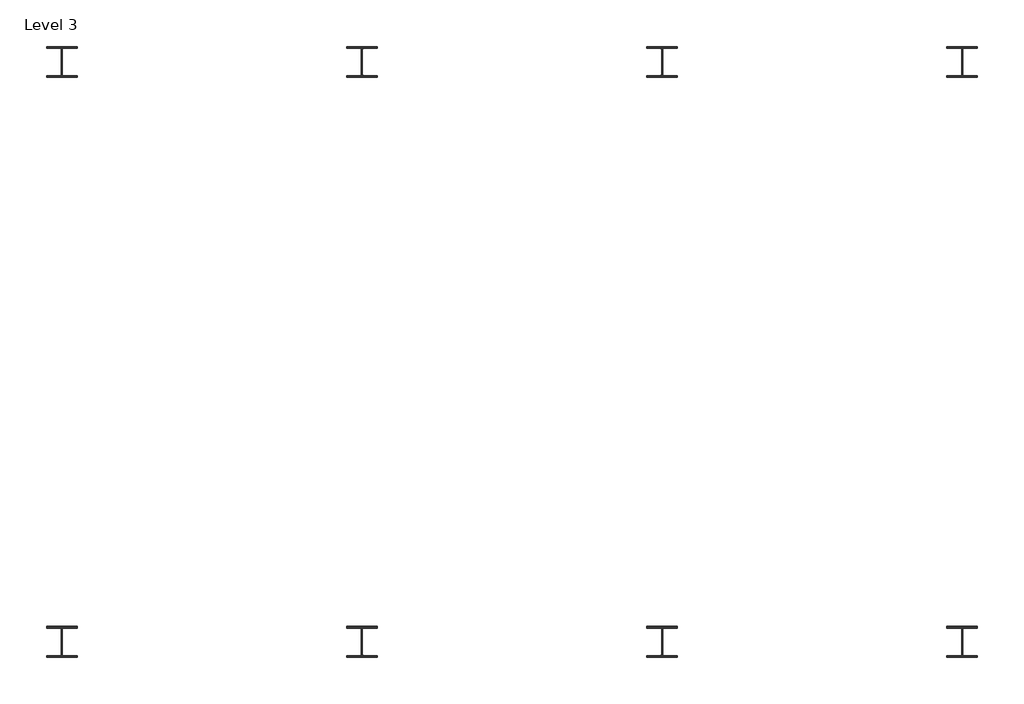
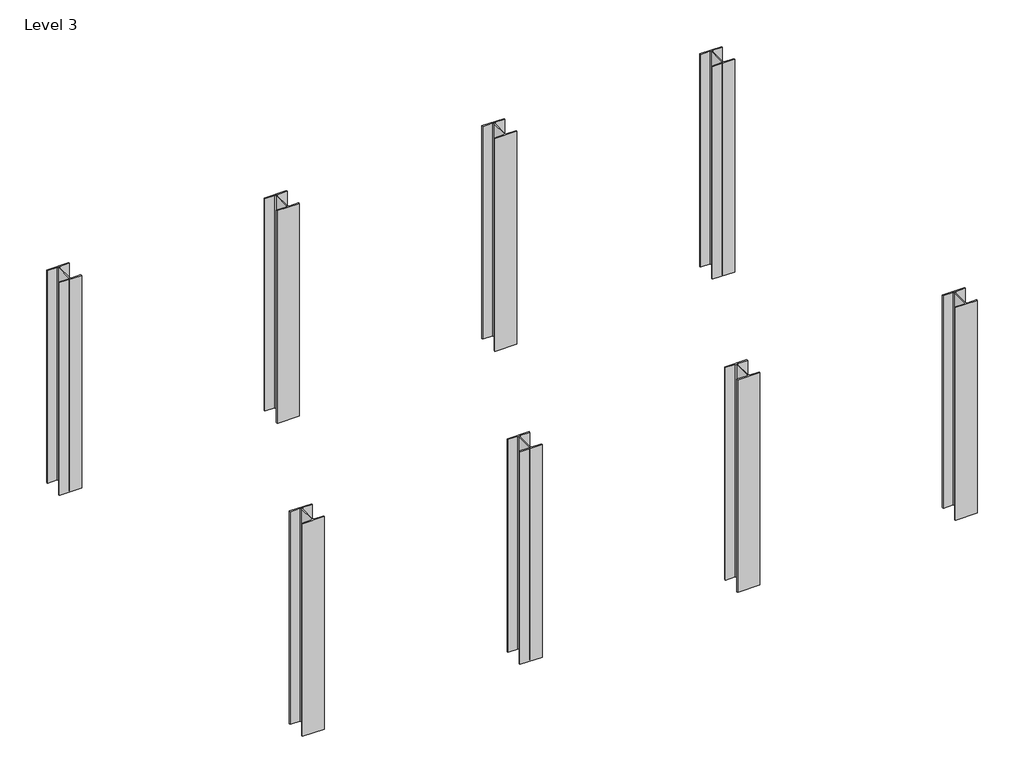
# One storey: 8 columns.
"""IFC4 building model written with IfcOpenShell, lengths in millimetres."""

import ifcopenshell
import ifcopenshell.guid

model = None  # the IFC model being written
_history = None  # IfcOwnerHistory: only IFC2X3 demands one
_inside = {}  # id of a spatial element -> (the spatial element, [elements in it])
_under = {}  # id of a project, library or spatial element -> (it, [spatial elements below it])
_declared = {}  # id of a project -> (the project, [libraries it declares])
_typed = {}  # id of a type object -> (the type object, [elements of that type])
_made_of = {}  # id of a material, layer set ... -> (it, [elements and type objects made of it])


def new_model(schema):
    """Start an empty IFC model of exactly this schema.

    Asked for "IFC4X3", IfcOpenShell would pick the latest addendum, in which some entities
    have other attributes; the version numbers below select the first issue.
    IFC2X3 requires an IfcOwnerHistory on every rooted entity: one is made here for all.
    """
    global model, _history
    if schema == "IFC4X3":
        model = ifcopenshell.file(schema_version=(4, 3, 0, 0))
    else:
        model = ifcopenshell.file(schema=schema)
    _inside.clear()
    _under.clear()
    _declared.clear()
    _typed.clear()
    _made_of.clear()
    _history = None
    if model.schema == "IFC2X3":
        org = make("IfcOrganization", Name="unknown")
        user = make(
            "IfcPersonAndOrganization",
            ThePerson=make("IfcPerson", FamilyName="unknown"),
            TheOrganization=org,
        )
        app = make(
            "IfcApplication",
            ApplicationDeveloper=org,
            Version="unknown",
            ApplicationFullName="unknown",
            ApplicationIdentifier="unknown",
        )
        _history = make(
            "IfcOwnerHistory",
            OwningUser=user,
            OwningApplication=app,
            ChangeAction="ADDED",
            CreationDate=0,
        )
    return model


def make(cls, **values):
    """One entity of the class cls with the attributes given. An attribute that is None is left unset."""
    return model.create_entity(
        cls, **{name: value for name, value in values.items() if value is not None}
    )


def rooted(cls, **values):
    """An entity with a GlobalId (a new one), such as an element, a storey or a relation."""
    return make(cls, GlobalId=ifcopenshell.guid.new(), OwnerHistory=_history, **values)


def si_unit(unit_type, name, prefix=None):
    """IfcSIUnit, for example si_unit("LENGTHUNIT", "METRE", prefix="MILLI")."""
    return make("IfcSIUnit", UnitType=unit_type, Prefix=prefix, Name=name)


def assignment(units):
    """IfcUnitAssignment: the units of a project."""
    return None if units is None else make("IfcUnitAssignment", Units=units)


def point(xyz):
    """IfcCartesianPoint."""
    return None if xyz is None else make("IfcCartesianPoint", Coordinates=xyz)


def direction(xyz):
    """IfcDirection."""
    return None if xyz is None else make("IfcDirection", DirectionRatios=xyz)


def frame(location, z_axis=None, x_axis=None):
    """IfcAxis2Placement3D, a coordinate frame: its origin and axes. An axis left out is left unset."""
    return make(
        "IfcAxis2Placement3D",
        Location=point(location),
        Axis=direction(z_axis),
        RefDirection=direction(x_axis),
    )


def frame_2d(location, x_axis=None):
    """IfcAxis2Placement2D, a coordinate frame in the plane: its origin and x axis."""
    return make(
        "IfcAxis2Placement2D", Location=point(location), RefDirection=direction(x_axis)
    )


def origin():
    """The frame at (0, 0, 0) with its axes left unset."""
    return frame((0.0, 0.0, 0.0))


def place(relative_to, where):
    """IfcLocalPlacement: puts the frame where relative to a parent placement (None: the world)."""
    return make(
        "IfcLocalPlacement", PlacementRelTo=relative_to, RelativePlacement=where
    )


def context(
    kind, dimensions, precision=None, world=None, true_north=None, identifier=None
):
    """IfcGeometricRepresentationContext, for example the 3D "Model" context."""
    return make(
        "IfcGeometricRepresentationContext",
        ContextIdentifier=identifier,
        ContextType=kind,
        CoordinateSpaceDimension=dimensions,
        Precision=precision,
        WorldCoordinateSystem=world,
        TrueNorth=true_north,
    )


def project(units=None, contexts=None):
    """IfcProject with its units and contexts."""
    return rooted(
        "IfcProject",
        Name="project",
        RepresentationContexts=contexts,
        UnitsInContext=assignment(units),
    )


def spatial(cls, under=None, at=None, **own):
    """A site, building, storey or space (cls), placed at a placement, below another one or the project."""
    s = rooted(cls, ObjectPlacement=at, **own)
    if under is not None:
        _under.setdefault(under.id(), (under, []))[1].append(s)
    return s


def polyline(points):
    """IfcPolyline through the points."""
    return make("IfcPolyline", Points=[point(p) for p in points])


def circle_curve(where, radius):
    """IfcCircle in the frame where."""
    return make("IfcCircle", Position=where, Radius=radius)


def trimmed(basis, trim1, trim2, sense, master):
    """IfcTrimmedCurve: the piece of a basis curve between two trims."""
    return make(
        "IfcTrimmedCurve",
        BasisCurve=basis,
        Trim1=trim1,
        Trim2=trim2,
        SenseAgreement=sense,
        MasterRepresentation=master,
    )


def segment(curve, same_sense, transition):
    """IfcCompositeCurveSegment."""
    return make(
        "IfcCompositeCurveSegment",
        Transition=transition,
        SameSense=same_sense,
        ParentCurve=curve,
    )


def composite_curve(segments, self_intersect=None):
    """IfcCompositeCurve: segments joined end to end."""
    return make("IfcCompositeCurve", Segments=segments, SelfIntersect=self_intersect)


def outline(outer, holes=None, kind="AREA"):
    """IfcArbitraryClosedProfileDef: a profile drawn as a closed curve; with holes, ...WithVoids."""
    if holes is None:
        return make("IfcArbitraryClosedProfileDef", ProfileType=kind, OuterCurve=outer)
    return make(
        "IfcArbitraryProfileDefWithVoids",
        ProfileType=kind,
        OuterCurve=outer,
        InnerCurves=holes,
    )


def extrude(swept, where, along, depth):
    """IfcExtrudedAreaSolid: the profile swept, set in the frame where, extruded along a direction by depth."""
    return make(
        "IfcExtrudedAreaSolid",
        SweptArea=swept,
        Position=where,
        ExtrudedDirection=direction(along),
        Depth=depth,
    )


def shape(context_of_items, identifier, shape_type, items):
    """IfcShapeRepresentation: the items that make up one representation, for example the "Body"."""
    return make(
        "IfcShapeRepresentation",
        ContextOfItems=context_of_items,
        RepresentationIdentifier=identifier,
        RepresentationType=shape_type,
        Items=items,
    )


def source(mapping_origin, context_of_items, identifier, shape_type, items):
    """IfcRepresentationMap: a shape defined once, which mapped items show again and again."""
    return make(
        "IfcRepresentationMap",
        MappingOrigin=mapping_origin,
        MappedRepresentation=shape(context_of_items, identifier, shape_type, items),
    )


def transform(
    local_origin,
    x_axis=None,
    y_axis=None,
    z_axis=None,
    scale=None,
    scale2=None,
    scale3=None,
    uniform=True,
):
    """IfcCartesianTransformationOperator3D, or its non-uniform kind. x_axis, y_axis, z_axis: its Axis1, 2, 3."""
    if uniform:
        return make(
            "IfcCartesianTransformationOperator3D",
            Axis1=direction(x_axis),
            Axis2=direction(y_axis),
            LocalOrigin=point(local_origin),
            Scale=scale,
            Axis3=direction(z_axis),
        )
    return make(
        "IfcCartesianTransformationOperator3DnonUniform",
        Axis1=direction(x_axis),
        Axis2=direction(y_axis),
        LocalOrigin=point(local_origin),
        Scale=scale,
        Axis3=direction(z_axis),
        Scale2=scale2,
        Scale3=scale3,
    )


def mapped(mapping_source, mapping_target):
    """IfcMappedItem: shows the shape of a source again, moved by a transform."""
    return make(
        "IfcMappedItem", MappingSource=mapping_source, MappingTarget=mapping_target
    )


def made_of(thing, what):
    """Note that an element or type object is made of a material, layer set ...; save() writes the relation."""
    if what is not None:
        _made_of.setdefault(what.id(), (what, []))[1].append(thing)
    return thing


def element(
    cls,
    number,
    at=None,
    inside=None,
    cuts=None,
    type_object=None,
    material=None,
    context=None,
    identifier="Body",
    shape_type=None,
    held_by="IfcProductDefinitionShape",
    body=None,
    shapes=None,
    **own,
):
    """One element of the class cls, such as IfcWall. Its Tag is "e" and its number.

    at: its placement. inside: the storey or other place that contains it. cuts: it is an
    opening in that element (IfcRelVoidsElement). A single representation is given by context,
    identifier, shape_type and body (its items); several are given by shapes. held_by: the class
    of the entity that holds the representations. save() writes the other relations.
    """
    e = rooted(cls, Tag="e%d" % number, ObjectPlacement=at, **own)
    if body is not None:
        shapes = [shape(context, identifier, shape_type, body)]
    if shapes is not None:
        e.Representation = make(held_by, Representations=shapes)
    if inside is not None:
        _inside.setdefault(inside.id(), (inside, []))[1].append(e)
    if cuts is not None:
        rooted(
            "IfcRelVoidsElement", RelatingBuildingElement=cuts, RelatedOpeningElement=e
        )
    if type_object is not None:
        _typed.setdefault(type_object.id(), (type_object, []))[1].append(e)
    return made_of(e, material)


def aggregate(whole, parts):
    """IfcRelAggregates: a whole, such as a stair, and the parts it consists of."""
    return rooted("IfcRelAggregates", RelatingObject=whole, RelatedObjects=parts)


def save(model, path):
    """Write the relations noted so far, then the file.

    IfcRelAggregates (storeys below a building ...), IfcRelContainedInSpatialStructure (elements
    in a storey), IfcRelDefinesByType, IfcRelAssociatesMaterial and IfcRelDeclares: one each for
    every whole, place, type object, material and project.
    """
    for whole, parts in _under.values():
        aggregate(whole, parts)
    for where, things in _inside.values():
        rooted(
            "IfcRelContainedInSpatialStructure",
            RelatedElements=things,
            RelatingStructure=where,
        )
    for kind, things in _typed.values():
        rooted("IfcRelDefinesByType", RelatedObjects=things, RelatingType=kind)
    for what, things in _made_of.values():
        rooted("IfcRelAssociatesMaterial", RelatedObjects=things, RelatingMaterial=what)
    for by, libraries in _declared.values():
        rooted("IfcRelDeclares", RelatingContext=by, RelatedDefinitions=libraries)
    model.write(path)


def uc_universal_columns_column_uc305x305x97_b067ee91(model_context):
    return source(origin(), model_context, "Body", "SweptSolid", [
        extrude(outline(composite_curve([segment(polyline([(152.65, 153.95), (152.65, 138.55), (20.15, 138.55)]), True, "CONTINUOUS"), segment(trimmed(circle_curve(frame_2d((20.15, 123.35)), 15.2), [point((20.15, 138.55))], [point((4.95, 123.35))], True, "CARTESIAN"), True, "CONTINUOUS"), segment(polyline([(4.95, 123.35), (4.95, -123.35)]), True, "CONTINUOUS"), segment(trimmed(circle_curve(frame_2d((20.15, -123.35)), 15.2), [point((4.95, -123.35))], [point((20.15, -138.55))], True, "CARTESIAN"), True, "CONTINUOUS"), segment(polyline([(20.15, -138.55), (152.65, -138.55), (152.65, -153.95), (-152.65, -153.95), (-152.65, -138.55), (-20.15, -138.55)]), True, "CONTINUOUS"), segment(trimmed(circle_curve(frame_2d((-20.15, -123.35)), 15.2), [point((-20.15, -138.55))], [point((-4.95, -123.35))], True, "CARTESIAN"), True, "CONTINUOUS"), segment(polyline([(-4.95, -123.35), (-4.95, 123.35)]), True, "CONTINUOUS"), segment(trimmed(circle_curve(frame_2d((-20.15, 123.35)), 15.2), [point((-4.95, 123.35))], [point((-20.15, 138.55))], True, "CARTESIAN"), True, "CONTINUOUS"), segment(polyline([(-20.15, 138.55), (-152.65, 138.55), (-152.65, 153.95), (152.65, 153.95)]), True, "CONTINUOUS")], self_intersect=False)), frame((0.0, 0.0, 2900.0), z_axis=(0.0, 0.0, 1.0), x_axis=(1.0, 0.0, 0.0)), (0.0, 0.0, 1.0), 3100.0),
    ])


model = new_model("IFC4")

# Units and contexts
model_context = context("Model", 3, world=origin())
ifc_project = project(units=[si_unit("LENGTHUNIT", "METRE", prefix="MILLI")], contexts=[model_context])

# Site, building, storey
site = spatial("IfcSite", under=ifc_project)
building = spatial("IfcBuilding", under=site)
storey = spatial("IfcBuildingStorey", under=building, Name="Level 3", Elevation=3000.0)

# Columns
placement = place(None, origin())
uc_universal_columns_column_uc305x305x97_shape = uc_universal_columns_column_uc305x305x97_b067ee91(model_context)
element("IfcColumn", 1, ObjectType="UC-Universal Columns-Column : UC305x305x97", at=placement, inside=storey, context=model_context, shape_type="MappedRepresentation", body=[
    mapped(uc_universal_columns_column_uc305x305x97_shape, transform((-1938.0684826, 2696.9060214, 0.0), x_axis=(-1.0, 0.0, 0.0), y_axis=(0.0, -1.0, 0.0), z_axis=(0.0, 0.0, 1.0))),
])
element("IfcColumn", 2, ObjectType="UC-Universal Columns-Column : UC305x305x97", at=placement, inside=storey, context=model_context, shape_type="MappedRepresentation", body=[
    mapped(uc_universal_columns_column_uc305x305x97_shape, transform((-1938.0684826, -3100.0939786, 0.0), x_axis=(-1.0, 0.0, 0.0), y_axis=(0.0, -1.0, 0.0), z_axis=(0.0, 0.0, 1.0))),
])
element("IfcColumn", 3, ObjectType="UC-Universal Columns-Column : UC305x305x97", at=placement, inside=storey, context=model_context, shape_type="MappedRepresentation", body=[
    mapped(uc_universal_columns_column_uc305x305x97_shape, transform((1061.9315174, 2696.9060214, 0.0), x_axis=(-1.0, 0.0, 0.0), y_axis=(0.0, -1.0, 0.0), z_axis=(0.0, 0.0, 1.0))),
])
element("IfcColumn", 4, ObjectType="UC-Universal Columns-Column : UC305x305x97", at=placement, inside=storey, context=model_context, shape_type="MappedRepresentation", body=[
    mapped(uc_universal_columns_column_uc305x305x97_shape, transform((1061.9315174, -3100.0939786, 0.0), x_axis=(-1.0, 0.0, 0.0), y_axis=(0.0, -1.0, 0.0), z_axis=(0.0, 0.0, 1.0))),
])
element("IfcColumn", 5, ObjectType="UC-Universal Columns-Column : UC305x305x97", at=placement, inside=storey, context=model_context, shape_type="MappedRepresentation", body=[
    mapped(uc_universal_columns_column_uc305x305x97_shape, transform((-4938.0684826, 2696.9060214, 0.0), x_axis=(-1.0, 0.0, 0.0), y_axis=(0.0, -1.0, 0.0), z_axis=(0.0, 0.0, 1.0))),
])
element("IfcColumn", 6, ObjectType="UC-Universal Columns-Column : UC305x305x97", at=placement, inside=storey, context=model_context, shape_type="MappedRepresentation", body=[
    mapped(uc_universal_columns_column_uc305x305x97_shape, transform((-4938.0684826, -3100.0939786, 0.0), x_axis=(-1.0, 0.0, 0.0), y_axis=(0.0, -1.0, 0.0), z_axis=(0.0, 0.0, 1.0))),
])
element("IfcColumn", 7, ObjectType="UC-Universal Columns-Column : UC305x305x97", at=placement, inside=storey, context=model_context, shape_type="MappedRepresentation", body=[
    mapped(uc_universal_columns_column_uc305x305x97_shape, transform((4061.9315174, 2696.9060214, 0.0), x_axis=(-1.0, 0.0, 0.0), y_axis=(0.0, -1.0, 0.0), z_axis=(0.0, 0.0, 1.0))),
])
element("IfcColumn", 8, ObjectType="UC-Universal Columns-Column : UC305x305x97", at=placement, inside=storey, context=model_context, shape_type="MappedRepresentation", body=[
    mapped(uc_universal_columns_column_uc305x305x97_shape, transform((4061.9315174, -3100.0939786, 0.0), x_axis=(-1.0, 0.0, 0.0), y_axis=(0.0, -1.0, 0.0), z_axis=(0.0, 0.0, 1.0))),
])

save(model, "model.ifc")

# Revit data of these elements
# Type "UC-Universal Columns-Column : UC305x305x97"
#   Section Name Key = "UC305x305x97"
#   Cost = 5
#   Width = 30.53 cm
#   Web Thickness = 0.99 cm
#   Web Fillet = 1.52 cm
#   Warping Constant = 1560000.0 cm⁶
#   Torsional Moment of Inertia = 91.20 cm⁴
#   Section Area = 123.0 cm²
#   Plastic Modulus weak axis = 726.0 cm³
#   Plastic Modulus strong axis = 1592.0 cm³
#   Nominal Weight = 96.8996 kgf/m
#   Moment of Inertia weak axis = 7308.00 cm⁴
#   Moment of Inertia strong axis = 22249.00 cm⁴
#   Height = 30.79 cm
#   Flange Thickness = 1.54 cm
#   Elastic Modulus weak axis = 479.0 cm³
#   Elastic Modulus strong axis = 1445.0 cm³
#   Centroid Vertical = 15.395 cm
#   Centroid Horizontal = 15.265 cm
#   Bolt Spacing = 14.0 cm
#   Structural Material [instance default] = Metal - Steel 43-275
#   Type Comments = ""
#   Assembly Code = ""
# Elements 1, 2, 3, 4, 5, 6, 7, 8 (IfcColumn, "UC-Universal Columns-Column : UC305x305x97")
#   Structural Material = Metal - Steel 43-275
#   Phase Created = New Construction
#   Materials on its faces: "Metal - Steel 43-275"
# Materials
#   "Metal - Steel 43-275": class "Metal", colour RGB 247 247 247, transparency 0, Cost = 0
